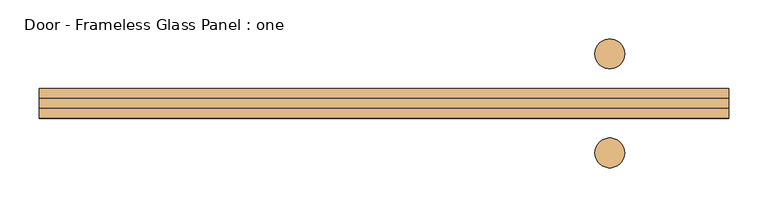
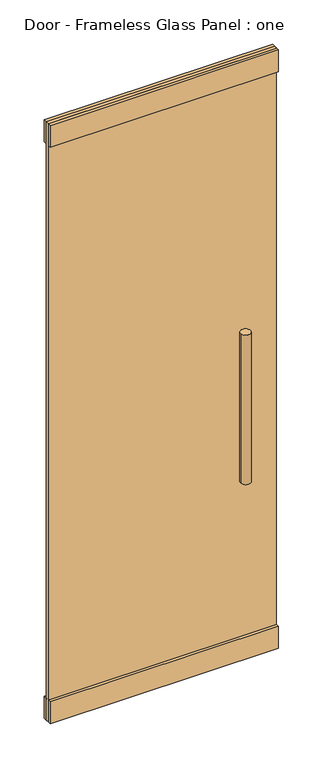
"""IFC4 building model written with IfcOpenShell, lengths in millimetres: door geometry, Door - Frameless Glass Panel : one."""

import ifcopenshell
import ifcopenshell.guid

model = None  # the IFC model being written
_history = None  # IfcOwnerHistory: only IFC2X3 demands one
_inside = {}  # id of a spatial element -> (the spatial element, [elements in it])
_under = {}  # id of a project, library or spatial element -> (it, [spatial elements below it])
_declared = {}  # id of a project -> (the project, [libraries it declares])
_typed = {}  # id of a type object -> (the type object, [elements of that type])
_made_of = {}  # id of a material, layer set ... -> (it, [elements and type objects made of it])


def new_model(schema):
    """Start an empty IFC model of exactly this schema.

    Asked for "IFC4X3", IfcOpenShell would pick the latest addendum, in which some entities
    have other attributes; the version numbers below select the first issue.
    IFC2X3 requires an IfcOwnerHistory on every rooted entity: one is made here for all.
    """
    global model, _history
    if schema == "IFC4X3":
        model = ifcopenshell.file(schema_version=(4, 3, 0, 0))
    else:
        model = ifcopenshell.file(schema=schema)
    _inside.clear()
    _under.clear()
    _declared.clear()
    _typed.clear()
    _made_of.clear()
    _history = None
    if model.schema == "IFC2X3":
        org = make("IfcOrganization", Name="unknown")
        user = make(
            "IfcPersonAndOrganization",
            ThePerson=make("IfcPerson", FamilyName="unknown"),
            TheOrganization=org,
        )
        app = make(
            "IfcApplication",
            ApplicationDeveloper=org,
            Version="unknown",
            ApplicationFullName="unknown",
            ApplicationIdentifier="unknown",
        )
        _history = make(
            "IfcOwnerHistory",
            OwningUser=user,
            OwningApplication=app,
            ChangeAction="ADDED",
            CreationDate=0,
        )
    return model


def make(cls, **values):
    """One entity of the class cls with the attributes given. An attribute that is None is left unset."""
    return model.create_entity(
        cls, **{name: value for name, value in values.items() if value is not None}
    )


def rooted(cls, **values):
    """An entity with a GlobalId (a new one), such as an element, a storey or a relation."""
    return make(cls, GlobalId=ifcopenshell.guid.new(), OwnerHistory=_history, **values)


def si_unit(unit_type, name, prefix=None):
    """IfcSIUnit, for example si_unit("LENGTHUNIT", "METRE", prefix="MILLI")."""
    return make("IfcSIUnit", UnitType=unit_type, Prefix=prefix, Name=name)


def assignment(units):
    """IfcUnitAssignment: the units of a project."""
    return None if units is None else make("IfcUnitAssignment", Units=units)


def point(xyz):
    """IfcCartesianPoint."""
    return None if xyz is None else make("IfcCartesianPoint", Coordinates=xyz)


def direction(xyz):
    """IfcDirection."""
    return None if xyz is None else make("IfcDirection", DirectionRatios=xyz)


def frame(location, z_axis=None, x_axis=None):
    """IfcAxis2Placement3D, a coordinate frame: its origin and axes. An axis left out is left unset."""
    return make(
        "IfcAxis2Placement3D",
        Location=point(location),
        Axis=direction(z_axis),
        RefDirection=direction(x_axis),
    )


def frame_2d(location, x_axis=None):
    """IfcAxis2Placement2D, a coordinate frame in the plane: its origin and x axis."""
    return make(
        "IfcAxis2Placement2D", Location=point(location), RefDirection=direction(x_axis)
    )


def origin():
    """The frame at (0, 0, 0) with its axes left unset."""
    return frame((0.0, 0.0, 0.0))


def origin_with_axes():
    """The frame at (0, 0, 0) with the z axis (0, 0, 1) and the x axis (1, 0, 0) written out."""
    return frame((0.0, 0.0, 0.0), z_axis=(0.0, 0.0, 1.0), x_axis=(1.0, 0.0, 0.0))


def place(relative_to, where):
    """IfcLocalPlacement: puts the frame where relative to a parent placement (None: the world)."""
    return make(
        "IfcLocalPlacement", PlacementRelTo=relative_to, RelativePlacement=where
    )


def context(
    kind, dimensions, precision=None, world=None, true_north=None, identifier=None
):
    """IfcGeometricRepresentationContext, for example the 3D "Model" context."""
    return make(
        "IfcGeometricRepresentationContext",
        ContextIdentifier=identifier,
        ContextType=kind,
        CoordinateSpaceDimension=dimensions,
        Precision=precision,
        WorldCoordinateSystem=world,
        TrueNorth=true_north,
    )


def project(units=None, contexts=None):
    """IfcProject with its units and contexts."""
    return rooted(
        "IfcProject",
        Name="project",
        RepresentationContexts=contexts,
        UnitsInContext=assignment(units),
    )


def spatial(cls, under=None, at=None, **own):
    """A site, building, storey or space (cls), placed at a placement, below another one or the project."""
    s = rooted(cls, ObjectPlacement=at, **own)
    if under is not None:
        _under.setdefault(under.id(), (under, []))[1].append(s)
    return s


def polyline(points):
    """IfcPolyline through the points."""
    return make("IfcPolyline", Points=[point(p) for p in points])


def circle_curve(where, radius):
    """IfcCircle in the frame where."""
    return make("IfcCircle", Position=where, Radius=radius)


def trimmed(basis, trim1, trim2, sense, master):
    """IfcTrimmedCurve: the piece of a basis curve between two trims."""
    return make(
        "IfcTrimmedCurve",
        BasisCurve=basis,
        Trim1=trim1,
        Trim2=trim2,
        SenseAgreement=sense,
        MasterRepresentation=master,
    )


def segment(curve, same_sense, transition):
    """IfcCompositeCurveSegment."""
    return make(
        "IfcCompositeCurveSegment",
        Transition=transition,
        SameSense=same_sense,
        ParentCurve=curve,
    )


def composite_curve(segments, self_intersect=None):
    """IfcCompositeCurve: segments joined end to end."""
    return make("IfcCompositeCurve", Segments=segments, SelfIntersect=self_intersect)


def outline(outer, holes=None, kind="AREA"):
    """IfcArbitraryClosedProfileDef: a profile drawn as a closed curve; with holes, ...WithVoids."""
    if holes is None:
        return make("IfcArbitraryClosedProfileDef", ProfileType=kind, OuterCurve=outer)
    return make(
        "IfcArbitraryProfileDefWithVoids",
        ProfileType=kind,
        OuterCurve=outer,
        InnerCurves=holes,
    )


def extrude(swept, where, along, depth):
    """IfcExtrudedAreaSolid: the profile swept, set in the frame where, extruded along a direction by depth."""
    return make(
        "IfcExtrudedAreaSolid",
        SweptArea=swept,
        Position=where,
        ExtrudedDirection=direction(along),
        Depth=depth,
    )


def shape(context_of_items, identifier, shape_type, items):
    """IfcShapeRepresentation: the items that make up one representation, for example the "Body"."""
    return make(
        "IfcShapeRepresentation",
        ContextOfItems=context_of_items,
        RepresentationIdentifier=identifier,
        RepresentationType=shape_type,
        Items=items,
    )


def source(mapping_origin, context_of_items, identifier, shape_type, items):
    """IfcRepresentationMap: a shape defined once, which mapped items show again and again."""
    return make(
        "IfcRepresentationMap",
        MappingOrigin=mapping_origin,
        MappedRepresentation=shape(context_of_items, identifier, shape_type, items),
    )


def transform(
    local_origin,
    x_axis=None,
    y_axis=None,
    z_axis=None,
    scale=None,
    scale2=None,
    scale3=None,
    uniform=True,
):
    """IfcCartesianTransformationOperator3D, or its non-uniform kind. x_axis, y_axis, z_axis: its Axis1, 2, 3."""
    if uniform:
        return make(
            "IfcCartesianTransformationOperator3D",
            Axis1=direction(x_axis),
            Axis2=direction(y_axis),
            LocalOrigin=point(local_origin),
            Scale=scale,
            Axis3=direction(z_axis),
        )
    return make(
        "IfcCartesianTransformationOperator3DnonUniform",
        Axis1=direction(x_axis),
        Axis2=direction(y_axis),
        LocalOrigin=point(local_origin),
        Scale=scale,
        Axis3=direction(z_axis),
        Scale2=scale2,
        Scale3=scale3,
    )


def mapped(mapping_source, mapping_target):
    """IfcMappedItem: shows the shape of a source again, moved by a transform."""
    return make(
        "IfcMappedItem", MappingSource=mapping_source, MappingTarget=mapping_target
    )


def made_of(thing, what):
    """Note that an element or type object is made of a material, layer set ...; save() writes the relation."""
    if what is not None:
        _made_of.setdefault(what.id(), (what, []))[1].append(thing)
    return thing


def element(
    cls,
    number,
    at=None,
    inside=None,
    cuts=None,
    type_object=None,
    material=None,
    context=None,
    identifier="Body",
    shape_type=None,
    held_by="IfcProductDefinitionShape",
    body=None,
    shapes=None,
    **own,
):
    """One element of the class cls, such as IfcWall. Its Tag is "e" and its number.

    at: its placement. inside: the storey or other place that contains it. cuts: it is an
    opening in that element (IfcRelVoidsElement). A single representation is given by context,
    identifier, shape_type and body (its items); several are given by shapes. held_by: the class
    of the entity that holds the representations. save() writes the other relations.
    """
    e = rooted(cls, Tag="e%d" % number, ObjectPlacement=at, **own)
    if body is not None:
        shapes = [shape(context, identifier, shape_type, body)]
    if shapes is not None:
        e.Representation = make(held_by, Representations=shapes)
    if inside is not None:
        _inside.setdefault(inside.id(), (inside, []))[1].append(e)
    if cuts is not None:
        rooted(
            "IfcRelVoidsElement", RelatingBuildingElement=cuts, RelatedOpeningElement=e
        )
    if type_object is not None:
        _typed.setdefault(type_object.id(), (type_object, []))[1].append(e)
    return made_of(e, material)


def aggregate(whole, parts):
    """IfcRelAggregates: a whole, such as a stair, and the parts it consists of."""
    return rooted("IfcRelAggregates", RelatingObject=whole, RelatedObjects=parts)


def save(model, path):
    """Write the relations noted so far, then the file.

    IfcRelAggregates (storeys below a building ...), IfcRelContainedInSpatialStructure (elements
    in a storey), IfcRelDefinesByType, IfcRelAssociatesMaterial and IfcRelDeclares: one each for
    every whole, place, type object, material and project.
    """
    for whole, parts in _under.values():
        aggregate(whole, parts)
    for where, things in _inside.values():
        rooted(
            "IfcRelContainedInSpatialStructure",
            RelatedElements=things,
            RelatingStructure=where,
        )
    for kind, things in _typed.values():
        rooted("IfcRelDefinesByType", RelatedObjects=things, RelatingType=kind)
    for what, things in _made_of.values():
        rooted("IfcRelAssociatesMaterial", RelatedObjects=things, RelatingMaterial=what)
    for by, libraries in _declared.values():
        rooted("IfcRelDeclares", RelatingContext=by, RelatedDefinitions=libraries)
    model.write(path)


def door_frameless_glass_panel_one_544ecd48(model_context):
    return source(origin(), model_context, "Body", "SweptSolid", [
        extrude(outline(composite_curve([segment(trimmed(circle_curve(frame_2d((288.925, 63.5)), 19.05), [point((269.875, 63.5))], [point((307.975, 63.5))], False, "CARTESIAN"), True, "CONTINUOUS"), segment(trimmed(circle_curve(frame_2d((288.925, 63.5)), 19.05), [point((307.975, 63.5))], [point((269.875, 63.5))], False, "CARTESIAN"), True, "CONTINUOUS")], self_intersect=False)), frame((0.0, 0.0, 762.0), z_axis=(0.0, 0.0, 1.0), x_axis=(1.0, 0.0, 0.0)), (0.0, 0.0, 1.0), 609.6),
        extrude(outline(composite_curve([segment(trimmed(circle_curve(frame_2d((288.925, -63.5)), 19.05), [point((269.875, -63.5))], [point((307.975, -63.5))], False, "CARTESIAN"), True, "CONTINUOUS"), segment(trimmed(circle_curve(frame_2d((288.925, -63.5)), 19.05), [point((307.975, -63.5))], [point((269.875, -63.5))], False, "CARTESIAN"), True, "CONTINUOUS")], self_intersect=False)), frame((0.0, 0.0, 762.0), z_axis=(0.0, 0.0, 1.0), x_axis=(1.0, 0.0, 0.0)), (0.0, 0.0, 1.0), 609.6),
        extrude(outline(polyline([(441.325, -6.35), (-441.325, -6.35), (-441.325, 6.35), (441.325, 6.35), (441.325, -6.35)])), origin_with_axes(), (0.0, 0.0, 1.0), 2444.75),
        extrude(outline(polyline([(-441.325, -19.05), (-441.325, 19.05), (441.325, 19.05), (441.325, -19.05), (-441.325, -19.05)])), origin_with_axes(), (0.0, 0.0, 1.0), 88.9),
        extrude(outline(polyline([(-441.325, -19.05), (-441.325, 19.05), (441.325, 19.05), (441.325, -19.05), (-441.325, -19.05)])), frame((0.0, 0.0, 2355.85), z_axis=(0.0, 0.0, 1.0), x_axis=(1.0, 0.0, 0.0)), (0.0, 0.0, 1.0), 88.9),
    ])


if __name__ == "__main__":
    model = new_model("IFC4")
    model_context = context("Model", 3, world=origin())
    ifc_project = project(units=[si_unit("LENGTHUNIT", "METRE", prefix="MILLI")], contexts=[model_context])
    site = spatial("IfcSite", under=ifc_project)
    building = spatial("IfcBuilding", under=site)
    placement = place(None, origin())
    door_frameless_glass_panel_one_shape = door_frameless_glass_panel_one_544ecd48(model_context)
    element("IfcDoor", 1, ObjectType="Door - Frameless Glass Panel : one", at=placement, inside=building, context=model_context, shape_type="MappedRepresentation", body=[
        mapped(door_frameless_glass_panel_one_shape, transform((0.0, 0.0, 0.0), x_axis=(1.0, 0.0, 0.0), y_axis=(0.0, 1.0, 0.0), z_axis=(0.0, 0.0, 1.0))),
    ])
    save(model, "model.ifc")

# Revit data of these elements
# Type "Door - Frameless Glass Panel : one"
#   Type Mark = "8"
#   Analytic Construction = "<None>"
#   Pivot Point [instance default] = 5' - 2.25212"
#   Glass Thickness = 0' - 0 1/2"
#   Gap btwn Panels = 0' - 0 1/4"
#   Panel Material = CLEAR TEMPERED GLASS (HEAD/SILL SUPPORT DETAILS TO MATCHING EXISTING FRAMLESS GLASS DETAILS @ TENANT ENTRANCE)
#   Handle Material = ALUM
# Element 1 (IfcDoor, "Door - Frameless Glass Panel : one")
#   Materials on its faces: "ALUM", "CLEAR TEMPERED GLASS (HEAD/SILL SUPPORT DETAILS TO MATCHING EXISTING FRAMLESS GLASS DETAILS @ TENANT ENTRANCE)"
# Materials
#   "CLEAR TEMPERED GLASS (HEAD/SILL SUPPORT DETAILS TO MATCHING EXISTING FRAMLESS GLASS DETAILS @ TENANT ENTRANCE)": class "Glass", colour RGB 218 227 224, transparency 1, Description = "Soda Lime Glass", Cost = 0
#   "ALUM": class "Generic", colour RGB 157 157 157, transparency 0, Cost = 0
